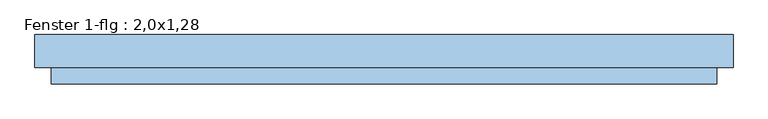
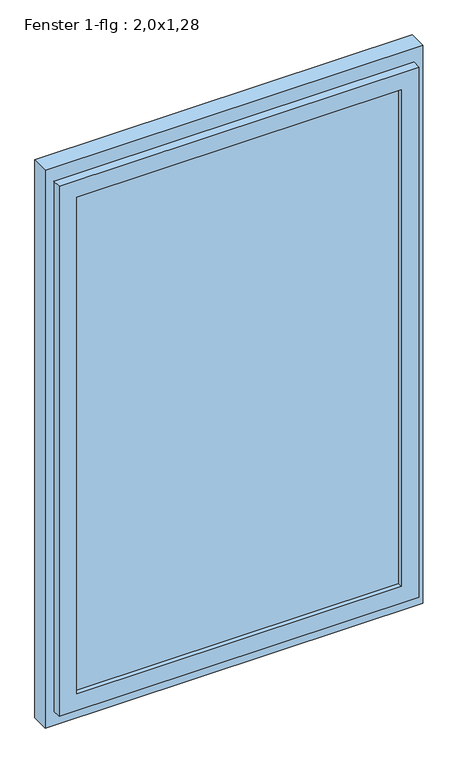
"""IFC4 building model written with IfcOpenShell, lengths in millimetres: window geometry, Fenster 1-flg : 2,0x1,28."""

from ifc_helpers import new_model, si_unit, frame, origin, place, context, project, spatial, polyline, outline, extrude, faceted_brep, source, transform, mapped, element, save


def fenster_1_flg_2_0x1_28_b67bdbe5(model_context):
    return source(origin(), model_context, "Body", "SolidModel", [
        extrude(outline(polyline([(3000.0, 640.0), (3000.0, -640.0), (1000.0, -640.0), (1000.0, 640.0), (3000.0, 640.0)]), holes=[polyline([(2920.0, 580.0), (1080.0, 580.0), (1080.0, -580.0), (2920.0, -580.0), (2920.0, 580.0)])]), frame((0.0, 20.0, 0.0), z_axis=(0.0, 1.0, 0.0), x_axis=(0.0, 0.0, 1.0)), (0.0, 0.0, 1.0), 60.0),
        faceted_brep([(610.0, 20.0, 2950.0), (610.0, -10.0, 2950.0), (610.0, -10.0, 1050.0), (610.0, 20.0, 1050.0), (-610.0, -10.0, 2950.0), (-610.0, -10.0, 1050.0), (550.0, -10.0, 1110.0), (-550.0, -10.0, 1110.0), (-550.0, -10.0, 2890.0), (550.0, -10.0, 2890.0), (-610.0, 20.0, 1050.0), (-610.0, 20.0, 2950.0), (580.0, 20.0, 2920.0), (-580.0, 20.0, 2920.0), (-580.0, 20.0, 1080.0), (580.0, 20.0, 1080.0), (580.0, 50.0, 2920.0), (580.0, 50.0, 1080.0), (-580.0, 50.0, 1080.0), (-580.0, 50.0, 2920.0), (550.0, 50.0, 2890.0), (-550.0, 50.0, 2890.0), (-550.0, 50.0, 1110.0), (550.0, 50.0, 1110.0)], [[[0, 1, 2, 3]], [[1, 4, 5, 2], [6, 7, 8, 9]], [[3, 2, 5, 10]], [[3, 10, 11, 0], [12, 13, 14, 15]], [[16, 12, 15, 17]], [[17, 15, 14, 18]], [[17, 18, 19, 16], [20, 21, 22, 23]], [[9, 20, 23, 6]], [[6, 23, 22, 7]], [[10, 5, 4, 11]], [[18, 14, 13, 19]], [[7, 22, 21, 8]], [[11, 4, 1, 0]], [[19, 13, 12, 16]], [[8, 21, 20, 9]]]),
        extrude(outline(polyline([(550.0, 5.0), (-550.0, 5.0), (-550.0, 35.0), (550.0, 35.0), (550.0, 5.0)])), frame((0.0, 0.0, 1110.0), z_axis=(0.0, 0.0, 1.0), x_axis=(1.0, 0.0, 0.0)), (0.0, 0.0, 1.0), 1780.0),
    ])


if __name__ == "__main__":
    model = new_model("IFC4")
    model_context = context("Model", 3, world=origin())
    ifc_project = project(units=[si_unit("LENGTHUNIT", "METRE", prefix="MILLI")], contexts=[model_context])
    site = spatial("IfcSite", under=ifc_project)
    building = spatial("IfcBuilding", under=site)
    placement = place(None, origin())
    fenster_1_flg_2_0x1_28_shape = fenster_1_flg_2_0x1_28_b67bdbe5(model_context)
    element("IfcWindow", 1, ObjectType="Fenster 1-flg : 2,0x1,28", at=placement, inside=building, context=model_context, shape_type="MappedRepresentation", body=[
        mapped(fenster_1_flg_2_0x1_28_shape, transform((0.0, 0.0, 0.0), x_axis=(1.0, 0.0, 0.0), y_axis=(0.0, 1.0, 0.0), z_axis=(0.0, 0.0, 1.0))),
    ])
    save(model, "model.ifc")

# Revit data of these elements
# Type "Fenster 1-flg : 2,0x1,28"
#   Type Mark = "64"
#   Operation = "SinglePanel"
#   Keynote = "16.05.01"
#   Visual Light Transmittance = 0.9
#   Solar Heat Gain Coefficient = 0.86
#   Rough Width = 1.280 m
#   Rough Height = 2.000 m
#   Heat Transfer Coefficient (U) = 5.5617 W/(m²·K)
#   Rahmentiefe = 0.060 m
#   Rahmenhöhe - unten = 0.080 m
#   Rahmenhöhe - oben = 0.080 m
#   Rahmenbreite = 0.060 m
#   Height = 2.000 m
#   Tiefe Flügel = 0.060 m
#   Flügelbreite = 0.060 m
#   Einbautiefe (von außen) [instance default] = 0.100 m
#   Width = 1.280 m
#   Klappflügel [instance default] = no
#   Kippflügel [instance default] = yes
#   Öffnungsrichtung in Draufsicht anzeigen [instance default] = no
#   Drehflügel 1 [instance default] = yes
#   Rahmen 1 [instance default] = none
#   Glas [instance default] = none
#   Flügel [instance default] = none
#   Fensterbank Innenseite [instance default] = none
#   Fensterbank Außenseite [instance default] = none
#   Construction Type Id = ""
#   Wall Closure = (empty or 0)
#   Analytic Construction = (empty or 0)
# Element 1 (IfcWindow, "Fenster 1-flg : 2,0x1,28")
#   Einbautiefe (von außen) = 0.230 m
#   Materials on its faces: "Kunststoff - Weiß", "Glas"
# Materials
#   "Kunststoff - Weiß": class "Kunststoff", colour RGB 249 249 249, transparency 0, Cost = 0
#   "Glas": class "Glas", colour RGB 0 0 255, transparency 0.75, Comments = "Render-Darstellung nicht aktualisiert ", Cost = 0
